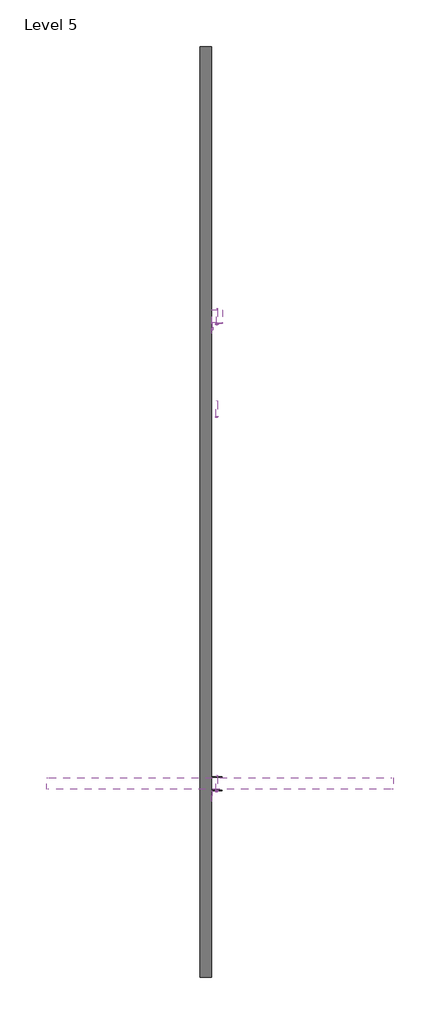
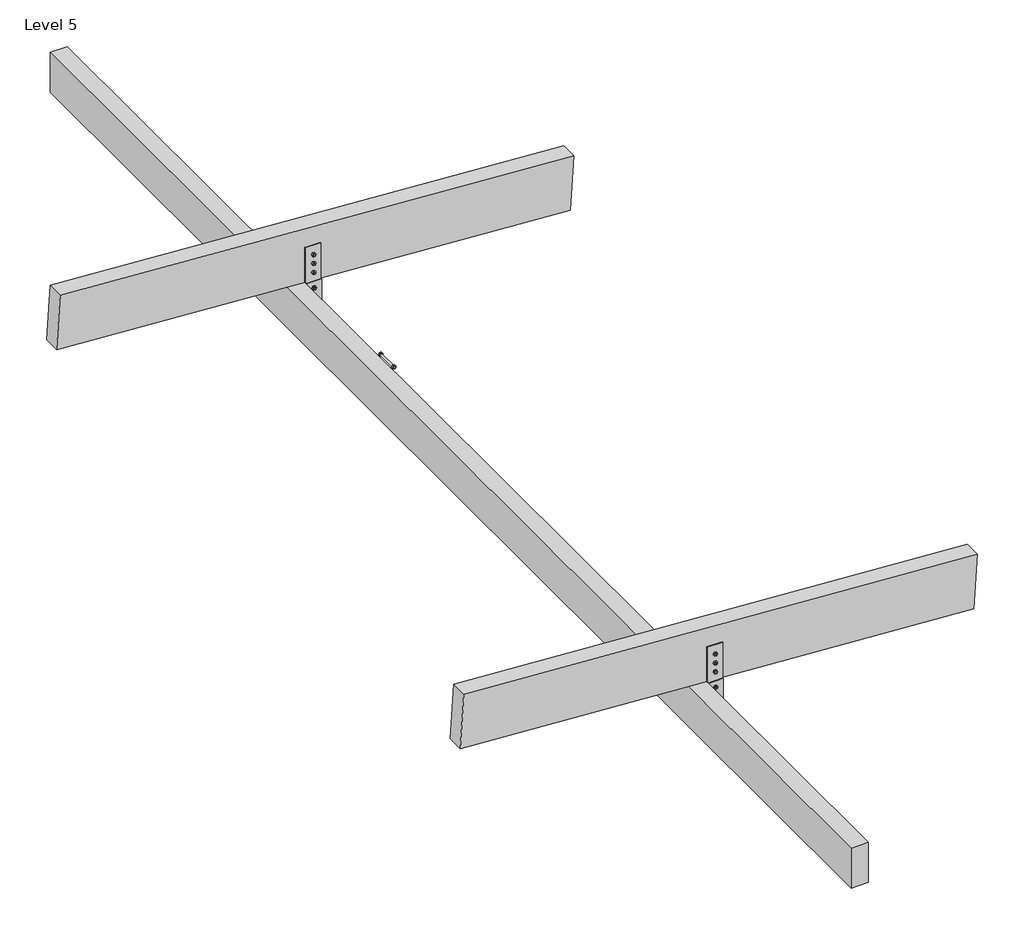
# One storey: 43 proxies.
"""IFC4 building model written with IfcOpenShell, lengths in millimetres."""

import ifcopenshell
import ifcopenshell.guid

model = None  # the IFC model being written
_history = None  # IfcOwnerHistory: only IFC2X3 demands one
_inside = {}  # id of a spatial element -> (the spatial element, [elements in it])
_under = {}  # id of a project, library or spatial element -> (it, [spatial elements below it])
_declared = {}  # id of a project -> (the project, [libraries it declares])
_typed = {}  # id of a type object -> (the type object, [elements of that type])
_made_of = {}  # id of a material, layer set ... -> (it, [elements and type objects made of it])


def new_model(schema):
    """Start an empty IFC model of exactly this schema.

    Asked for "IFC4X3", IfcOpenShell would pick the latest addendum, in which some entities
    have other attributes; the version numbers below select the first issue.
    IFC2X3 requires an IfcOwnerHistory on every rooted entity: one is made here for all.
    """
    global model, _history
    if schema == "IFC4X3":
        model = ifcopenshell.file(schema_version=(4, 3, 0, 0))
    else:
        model = ifcopenshell.file(schema=schema)
    _inside.clear()
    _under.clear()
    _declared.clear()
    _typed.clear()
    _made_of.clear()
    _history = None
    if model.schema == "IFC2X3":
        org = make("IfcOrganization", Name="unknown")
        user = make(
            "IfcPersonAndOrganization",
            ThePerson=make("IfcPerson", FamilyName="unknown"),
            TheOrganization=org,
        )
        app = make(
            "IfcApplication",
            ApplicationDeveloper=org,
            Version="unknown",
            ApplicationFullName="unknown",
            ApplicationIdentifier="unknown",
        )
        _history = make(
            "IfcOwnerHistory",
            OwningUser=user,
            OwningApplication=app,
            ChangeAction="ADDED",
            CreationDate=0,
        )
    return model


def make(cls, **values):
    """One entity of the class cls with the attributes given. An attribute that is None is left unset."""
    return model.create_entity(
        cls, **{name: value for name, value in values.items() if value is not None}
    )


def rooted(cls, **values):
    """An entity with a GlobalId (a new one), such as an element, a storey or a relation."""
    return make(cls, GlobalId=ifcopenshell.guid.new(), OwnerHistory=_history, **values)


def si_unit(unit_type, name, prefix=None):
    """IfcSIUnit, for example si_unit("LENGTHUNIT", "METRE", prefix="MILLI")."""
    return make("IfcSIUnit", UnitType=unit_type, Prefix=prefix, Name=name)


def assignment(units):
    """IfcUnitAssignment: the units of a project."""
    return None if units is None else make("IfcUnitAssignment", Units=units)


def point(xyz):
    """IfcCartesianPoint."""
    return None if xyz is None else make("IfcCartesianPoint", Coordinates=xyz)


def direction(xyz):
    """IfcDirection."""
    return None if xyz is None else make("IfcDirection", DirectionRatios=xyz)


def frame(location, z_axis=None, x_axis=None):
    """IfcAxis2Placement3D, a coordinate frame: its origin and axes. An axis left out is left unset."""
    return make(
        "IfcAxis2Placement3D",
        Location=point(location),
        Axis=direction(z_axis),
        RefDirection=direction(x_axis),
    )


def frame_2d(location, x_axis=None):
    """IfcAxis2Placement2D, a coordinate frame in the plane: its origin and x axis."""
    return make(
        "IfcAxis2Placement2D", Location=point(location), RefDirection=direction(x_axis)
    )


def origin():
    """The frame at (0, 0, 0) with its axes left unset."""
    return frame((0.0, 0.0, 0.0))


def origin_2d():
    """The frame at (0, 0) in the plane with its x axis left unset."""
    return frame_2d((0.0, 0.0))


def place(relative_to, where):
    """IfcLocalPlacement: puts the frame where relative to a parent placement (None: the world)."""
    return make(
        "IfcLocalPlacement", PlacementRelTo=relative_to, RelativePlacement=where
    )


def context(
    kind, dimensions, precision=None, world=None, true_north=None, identifier=None
):
    """IfcGeometricRepresentationContext, for example the 3D "Model" context."""
    return make(
        "IfcGeometricRepresentationContext",
        ContextIdentifier=identifier,
        ContextType=kind,
        CoordinateSpaceDimension=dimensions,
        Precision=precision,
        WorldCoordinateSystem=world,
        TrueNorth=true_north,
    )


def project(units=None, contexts=None):
    """IfcProject with its units and contexts."""
    return rooted(
        "IfcProject",
        Name="project",
        RepresentationContexts=contexts,
        UnitsInContext=assignment(units),
    )


def spatial(cls, under=None, at=None, **own):
    """A site, building, storey or space (cls), placed at a placement, below another one or the project."""
    s = rooted(cls, ObjectPlacement=at, **own)
    if under is not None:
        _under.setdefault(under.id(), (under, []))[1].append(s)
    return s


def polyline(points):
    """IfcPolyline through the points."""
    return make("IfcPolyline", Points=[point(p) for p in points])


def circle_curve(where, radius):
    """IfcCircle in the frame where."""
    return make("IfcCircle", Position=where, Radius=radius)


def trimmed(basis, trim1, trim2, sense, master):
    """IfcTrimmedCurve: the piece of a basis curve between two trims."""
    return make(
        "IfcTrimmedCurve",
        BasisCurve=basis,
        Trim1=trim1,
        Trim2=trim2,
        SenseAgreement=sense,
        MasterRepresentation=master,
    )


def segment(curve, same_sense, transition):
    """IfcCompositeCurveSegment."""
    return make(
        "IfcCompositeCurveSegment",
        Transition=transition,
        SameSense=same_sense,
        ParentCurve=curve,
    )


def composite_curve(segments, self_intersect=None):
    """IfcCompositeCurve: segments joined end to end."""
    return make("IfcCompositeCurve", Segments=segments, SelfIntersect=self_intersect)


def outline(outer, holes=None, kind="AREA"):
    """IfcArbitraryClosedProfileDef: a profile drawn as a closed curve; with holes, ...WithVoids."""
    if holes is None:
        return make("IfcArbitraryClosedProfileDef", ProfileType=kind, OuterCurve=outer)
    return make(
        "IfcArbitraryProfileDefWithVoids",
        ProfileType=kind,
        OuterCurve=outer,
        InnerCurves=holes,
    )


def extrude(swept, where, along, depth):
    """IfcExtrudedAreaSolid: the profile swept, set in the frame where, extruded along a direction by depth."""
    return make(
        "IfcExtrudedAreaSolid",
        SweptArea=swept,
        Position=where,
        ExtrudedDirection=direction(along),
        Depth=depth,
    )


def shape(context_of_items, identifier, shape_type, items):
    """IfcShapeRepresentation: the items that make up one representation, for example the "Body"."""
    return make(
        "IfcShapeRepresentation",
        ContextOfItems=context_of_items,
        RepresentationIdentifier=identifier,
        RepresentationType=shape_type,
        Items=items,
    )


def source(mapping_origin, context_of_items, identifier, shape_type, items):
    """IfcRepresentationMap: a shape defined once, which mapped items show again and again."""
    return make(
        "IfcRepresentationMap",
        MappingOrigin=mapping_origin,
        MappedRepresentation=shape(context_of_items, identifier, shape_type, items),
    )


def transform(
    local_origin,
    x_axis=None,
    y_axis=None,
    z_axis=None,
    scale=None,
    scale2=None,
    scale3=None,
    uniform=True,
):
    """IfcCartesianTransformationOperator3D, or its non-uniform kind. x_axis, y_axis, z_axis: its Axis1, 2, 3."""
    if uniform:
        return make(
            "IfcCartesianTransformationOperator3D",
            Axis1=direction(x_axis),
            Axis2=direction(y_axis),
            LocalOrigin=point(local_origin),
            Scale=scale,
            Axis3=direction(z_axis),
        )
    return make(
        "IfcCartesianTransformationOperator3DnonUniform",
        Axis1=direction(x_axis),
        Axis2=direction(y_axis),
        LocalOrigin=point(local_origin),
        Scale=scale,
        Axis3=direction(z_axis),
        Scale2=scale2,
        Scale3=scale3,
    )


def mapped(mapping_source, mapping_target):
    """IfcMappedItem: shows the shape of a source again, moved by a transform."""
    return make(
        "IfcMappedItem", MappingSource=mapping_source, MappingTarget=mapping_target
    )


def made_of(thing, what):
    """Note that an element or type object is made of a material, layer set ...; save() writes the relation."""
    if what is not None:
        _made_of.setdefault(what.id(), (what, []))[1].append(thing)
    return thing


def element(
    cls,
    number,
    at=None,
    inside=None,
    cuts=None,
    type_object=None,
    material=None,
    context=None,
    identifier="Body",
    shape_type=None,
    held_by="IfcProductDefinitionShape",
    body=None,
    shapes=None,
    **own,
):
    """One element of the class cls, such as IfcWall. Its Tag is "e" and its number.

    at: its placement. inside: the storey or other place that contains it. cuts: it is an
    opening in that element (IfcRelVoidsElement). A single representation is given by context,
    identifier, shape_type and body (its items); several are given by shapes. held_by: the class
    of the entity that holds the representations. save() writes the other relations.
    """
    e = rooted(cls, Tag="e%d" % number, ObjectPlacement=at, **own)
    if body is not None:
        shapes = [shape(context, identifier, shape_type, body)]
    if shapes is not None:
        e.Representation = make(held_by, Representations=shapes)
    if inside is not None:
        _inside.setdefault(inside.id(), (inside, []))[1].append(e)
    if cuts is not None:
        rooted(
            "IfcRelVoidsElement", RelatingBuildingElement=cuts, RelatedOpeningElement=e
        )
    if type_object is not None:
        _typed.setdefault(type_object.id(), (type_object, []))[1].append(e)
    return made_of(e, material)


def aggregate(whole, parts):
    """IfcRelAggregates: a whole, such as a stair, and the parts it consists of."""
    return rooted("IfcRelAggregates", RelatingObject=whole, RelatedObjects=parts)


def save(model, path):
    """Write the relations noted so far, then the file.

    IfcRelAggregates (storeys below a building ...), IfcRelContainedInSpatialStructure (elements
    in a storey), IfcRelDefinesByType, IfcRelAssociatesMaterial and IfcRelDeclares: one each for
    every whole, place, type object, material and project.
    """
    for whole, parts in _under.values():
        aggregate(whole, parts)
    for where, things in _inside.values():
        rooted(
            "IfcRelContainedInSpatialStructure",
            RelatedElements=things,
            RelatingStructure=where,
        )
    for kind, things in _typed.values():
        rooted("IfcRelDefinesByType", RelatedObjects=things, RelatingType=kind)
    for what, things in _made_of.values():
        rooted("IfcRelAssociatesMaterial", RelatedObjects=things, RelatingMaterial=what)
    for by, libraries in _declared.values():
        rooted("IfcRelDeclares", RelatingContext=by, RelatedDefinitions=libraries)
    model.write(path)


def generic_models_108_generic_models_73_f9342414(model_context):
    return source(origin(), model_context, "Body", "SweptSolid", [
        extrude(outline(polyline([(30850.5406612, 271789.525), (30698.1406612, 271789.525), (30698.1406612, 271383.125), (30690.2031612, 271383.125), (30690.2031612, 271797.4625), (30858.4781612, 271797.4625), (30858.4781612, 271383.125), (30850.5406612, 271383.125), (30850.5406612, 271789.525)])), frame((31923.0340778, 0.0, 0.0), z_axis=(1.0, 0.0, 0.0), x_axis=(0.0, 1.0, 0.0)), (0.0, 0.0, 1.0), 127.0),
    ])


def generic_models_142_generic_models_75_680a847f(model_context):
    return source(origin(), model_context, "Body", "SweptSolid", [
        extrude(outline(polyline([(271581.5625, 31979.8726858), (271581.5625, 31996.3704698), (271595.85, 32004.6193618), (271610.1375, 31996.3704698), (271610.1375, 31979.8726858), (271595.85, 31971.6237939), (271581.5625, 31979.8726858)])), frame((0.0, 36311.3770442, 0.0), z_axis=(0.0, 1.0, 0.0), x_axis=(0.0, 0.0, 1.0)), (0.0, 0.0, 1.0), 11.90625),
        extrude(outline(polyline([(271581.5625, 31979.8726858), (271581.5625, 31996.3704698), (271595.85, 32004.6193618), (271610.1375, 31996.3704698), (271610.1375, 31979.8726858), (271595.85, 31971.6237939), (271581.5625, 31979.8726858)])), frame((0.0, 36491.5582942, 0.0), z_axis=(0.0, 1.0, 0.0), x_axis=(0.0, 0.0, 1.0)), (0.0, 0.0, 1.0), 11.90625),
    ])


def generic_models_155_generic_models_75_12a366e2(model_context):
    return source(origin(), model_context, "Body", "SweptSolid", [
        extrude(outline(polyline([(271657.7625, 31979.8726858), (271657.7625, 31996.3704698), (271672.05, 32004.6193618), (271686.3375, 31996.3704698), (271686.3375, 31979.8726858), (271672.05, 31971.6237939), (271657.7625, 31979.8726858)])), frame((0.0, 36311.3770442, 0.0), z_axis=(0.0, 1.0, 0.0), x_axis=(0.0, 0.0, 1.0)), (0.0, 0.0, 1.0), 11.90625),
        extrude(outline(polyline([(271657.7625, 31979.8726858), (271657.7625, 31996.3704698), (271672.05, 32004.6193618), (271686.3375, 31996.3704698), (271686.3375, 31979.8726858), (271672.05, 31971.6237939), (271657.7625, 31979.8726858)])), frame((0.0, 36491.5582942, 0.0), z_axis=(0.0, 1.0, 0.0), x_axis=(0.0, 0.0, 1.0)), (0.0, 0.0, 1.0), 11.90625),
    ])


def generic_models_166_generic_models_73_e2e018fc(model_context):
    return source(origin(), model_context, "Body", "SweptSolid", [
        extrude(outline(polyline([(31923.0340778, 30690.2031612), (31930.9715778, 30690.2031612), (31930.9715778, 30563.2031612), (31923.0340778, 30563.2031612), (31923.0340778, 30690.2031612)])), frame((0.0, 0.0, 271490.7765953), z_axis=(0.0, 0.0, 1.0), x_axis=(1.0, 0.0, 0.0)), (0.0, 0.0, 1.0), 295.5734047),
        extrude(outline(polyline([(31923.0340778, 30985.4781612), (31930.9715778, 30985.4781612), (31930.9715778, 30858.4781612), (31923.0340778, 30858.4781612), (31923.0340778, 30985.4781612)])), frame((0.0, 0.0, 271490.7765953), z_axis=(0.0, 0.0, 1.0), x_axis=(1.0, 0.0, 0.0)), (0.0, 0.0, 1.0), 295.5734047),
        extrude(outline(polyline([(32050.0340778, 30852.1281612), (32050.0340778, 30844.1906612), (31923.0340778, 30844.1906612), (31923.0340778, 30852.1281612), (32050.0340778, 30852.1281612)])), frame((0.0, 0.0, 271797.4625), z_axis=(0.0, 0.0, 1.0), x_axis=(1.0, 0.0, 0.0)), (0.0, 0.0, 1.0), 306.5595065),
        extrude(outline(polyline([(32050.0340778, 30704.4906612), (32050.0340778, 30696.5531612), (31923.0340778, 30696.5531612), (31923.0340778, 30704.4906612), (32050.0340778, 30704.4906612)])), frame((0.0, 0.0, 271797.4625), z_axis=(0.0, 0.0, 1.0), x_axis=(1.0, 0.0, 0.0)), (0.0, 0.0, 1.0), 306.5595065),
    ])


def generic_models_168_generic_models_75_28256fc9(model_context):
    return source(origin(), model_context, "Body", "SweptSolid", [
        extrude(outline(polyline([(271505.3625, 31978.2851858), (271505.3625, 31994.7829698), (271519.65, 32003.0318618), (271533.9375, 31994.7829698), (271533.9375, 31978.2851858), (271519.65, 31970.0362939), (271505.3625, 31978.2851858)])), frame((0.0, 35193.7770442, 0.0), z_axis=(0.0, 1.0, 0.0), x_axis=(0.0, 0.0, 1.0)), (0.0, 0.0, 1.0), 11.90625),
        extrude(outline(polyline([(271505.3625, 31978.2851858), (271505.3625, 31994.7829698), (271519.65, 32003.0318618), (271533.9375, 31994.7829698), (271533.9375, 31978.2851858), (271519.65, 31970.0362939), (271505.3625, 31978.2851858)])), frame((0.0, 35373.9582942, 0.0), z_axis=(0.0, 1.0, 0.0), x_axis=(0.0, 0.0, 1.0)), (0.0, 0.0, 1.0), 11.90625),
    ])


def generic_models_172_generic_models_70_ead40be0(model_context):
    return source(origin(), model_context, "Body", "SweptSolid", [
        extrude(outline(polyline([(0.0, -4165.0140379), (0.0, 0.0), (139.7, 0.0), (139.7, -4165.0140379), (0.0, -4165.0140379)])), frame((29915.3947278, 36337.5707942, 271930.8774594), z_axis=(0.062378286155191545, 0.0, 0.9980525784828879), x_axis=(0.0, 1.0, 0.0)), (0.0, 0.0, 1.0), 457.2),
        extrude(outline(polyline([(0.0, -4165.0140379), (0.0, 0.0), (139.7, 0.0), (139.7, -4165.0140379), (0.0, -4165.0140379)])), frame((29929.8137808, 30704.4906612, 271929.9762686), z_axis=(0.06237828615519167, 0.0, 0.9980525784828879), x_axis=(0.0, 1.0, 0.0)), (0.0, 0.0, 1.0), 457.2),
    ])


def generic_models_173_generic_models_75_790f61a9(model_context):
    return source(origin(), model_context, "Body", "SweptSolid", [
        extrude(outline(polyline([(271581.5625, 31978.2851858), (271581.5625, 31994.7829698), (271595.85, 32003.0318618), (271610.1375, 31994.7829698), (271610.1375, 31978.2851858), (271595.85, 31970.0362939), (271581.5625, 31978.2851858)])), frame((0.0, 35193.7770442, 0.0), z_axis=(0.0, 1.0, 0.0), x_axis=(0.0, 0.0, 1.0)), (0.0, 0.0, 1.0), 11.90625),
        extrude(outline(polyline([(271581.5625, 31978.2851858), (271581.5625, 31994.7829698), (271595.85, 32003.0318618), (271610.1375, 31994.7829698), (271610.1375, 31978.2851858), (271595.85, 31970.0362939), (271581.5625, 31978.2851858)])), frame((0.0, 35373.9582942, 0.0), z_axis=(0.0, 1.0, 0.0), x_axis=(0.0, 0.0, 1.0)), (0.0, 0.0, 1.0), 11.90625),
    ])


def generic_models_174_generic_models_75_63e9463d(model_context):
    return source(origin(), model_context, "Body", "SweptSolid", [
        extrude(outline(polyline([(272027.8220065, 31970.0362939), (272013.5345065, 31978.2851858), (272013.5345065, 31994.7829698), (272027.8220065, 32003.0318618), (272042.1095065, 31994.7829698), (272042.1095065, 31978.2851858), (272027.8220065, 31970.0362939)])), frame((0.0, 30684.6469112, 0.0), z_axis=(0.0, 1.0, 0.0), x_axis=(0.0, 0.0, 1.0)), (0.0, 0.0, 1.0), 11.90625),
        extrude(outline(polyline([(272027.8220065, 31970.0362939), (272013.5345065, 31978.2851858), (272013.5345065, 31994.7829698), (272027.8220065, 32003.0318618), (272042.1095065, 31994.7829698), (272042.1095065, 31978.2851858), (272027.8220065, 31970.0362939)])), frame((0.0, 30852.1281612, 0.0), z_axis=(0.0, 1.0, 0.0), x_axis=(0.0, 0.0, 1.0)), (0.0, 0.0, 1.0), 11.90625),
        extrude(outline(polyline([(271951.6220065, 31970.0362939), (271937.3345065, 31978.2851858), (271937.3345065, 31994.7829698), (271951.6220065, 32003.0318618), (271965.9095065, 31994.7829698), (271965.9095065, 31978.2851858), (271951.6220065, 31970.0362939)])), frame((0.0, 30684.6469112, 0.0), z_axis=(0.0, 1.0, 0.0), x_axis=(0.0, 0.0, 1.0)), (0.0, 0.0, 1.0), 11.90625),
        extrude(outline(polyline([(271951.6220065, 31970.0362939), (271937.3345065, 31978.2851858), (271937.3345065, 31994.7829698), (271951.6220065, 32003.0318618), (271965.9095065, 31994.7829698), (271965.9095065, 31978.2851858), (271951.6220065, 31970.0362939)])), frame((0.0, 30852.1281612, 0.0), z_axis=(0.0, 1.0, 0.0), x_axis=(0.0, 0.0, 1.0)), (0.0, 0.0, 1.0), 11.90625),
        extrude(outline(polyline([(271875.4220065, 31970.0362939), (271861.1345065, 31978.2851858), (271861.1345065, 31994.7829698), (271875.4220065, 32003.0318618), (271889.7095065, 31994.7829698), (271889.7095065, 31978.2851858), (271875.4220065, 31970.0362939)])), frame((0.0, 30684.6469112, 0.0), z_axis=(0.0, 1.0, 0.0), x_axis=(0.0, 0.0, 1.0)), (0.0, 0.0, 1.0), 11.90625),
        extrude(outline(polyline([(271875.4220065, 31970.0362939), (271861.1345065, 31978.2851858), (271861.1345065, 31994.7829698), (271875.4220065, 32003.0318618), (271889.7095065, 31994.7829698), (271889.7095065, 31978.2851858), (271875.4220065, 31970.0362939)])), frame((0.0, 30852.1281612, 0.0), z_axis=(0.0, 1.0, 0.0), x_axis=(0.0, 0.0, 1.0)), (0.0, 0.0, 1.0), 11.90625),
    ])


def generic_models_175_generic_models_75_4c8c2855(model_context):
    return source(origin(), model_context, "Body", "SweptSolid", [
        extrude(outline(polyline([(271657.7625, 31978.2851858), (271657.7625, 31994.7829698), (271672.05, 32003.0318618), (271686.3375, 31994.7829698), (271686.3375, 31978.2851858), (271672.05, 31970.0362939), (271657.7625, 31978.2851858)])), frame((0.0, 35193.7770442, 0.0), z_axis=(0.0, 1.0, 0.0), x_axis=(0.0, 0.0, 1.0)), (0.0, 0.0, 1.0), 11.90625),
        extrude(outline(polyline([(271657.7625, 31978.2851858), (271657.7625, 31994.7829698), (271672.05, 32003.0318618), (271686.3375, 31994.7829698), (271686.3375, 31978.2851858), (271672.05, 31970.0362939), (271657.7625, 31978.2851858)])), frame((0.0, 35373.9582942, 0.0), z_axis=(0.0, 1.0, 0.0), x_axis=(0.0, 0.0, 1.0)), (0.0, 0.0, 1.0), 11.90625),
    ])


def generic_models_176_generic_models_75_eb76e51d(model_context):
    return source(origin(), model_context, "Body", "SweptSolid", [
        extrude(outline(polyline([(271733.9625, 31978.2851858), (271733.9625, 31994.7829698), (271748.25, 32003.0318618), (271762.5375, 31994.7829698), (271762.5375, 31978.2851858), (271748.25, 31970.0362939), (271733.9625, 31978.2851858)])), frame((0.0, 35193.7770442, 0.0), z_axis=(0.0, 1.0, 0.0), x_axis=(0.0, 0.0, 1.0)), (0.0, 0.0, 1.0), 11.90625),
        extrude(outline(polyline([(271733.9625, 31978.2851858), (271733.9625, 31994.7829698), (271748.25, 32003.0318618), (271762.5375, 31994.7829698), (271762.5375, 31978.2851858), (271748.25, 31970.0362939), (271733.9625, 31978.2851858)])), frame((0.0, 35373.9582942, 0.0), z_axis=(0.0, 1.0, 0.0), x_axis=(0.0, 0.0, 1.0)), (0.0, 0.0, 1.0), 11.90625),
    ])


def generic_models_179_generic_models_75_1166544c(model_context):
    return source(origin(), model_context, "Body", "SweptSolid", [
        extrude(outline(polyline([(271733.9625, 31979.8726858), (271733.9625, 31996.3704698), (271748.25, 32004.6193618), (271762.5375, 31996.3704698), (271762.5375, 31979.8726858), (271748.25, 31971.6237939), (271733.9625, 31979.8726858)])), frame((0.0, 36311.3770442, 0.0), z_axis=(0.0, 1.0, 0.0), x_axis=(0.0, 0.0, 1.0)), (0.0, 0.0, 1.0), 11.90625),
        extrude(outline(polyline([(271733.9625, 31979.8726858), (271733.9625, 31996.3704698), (271748.25, 32004.6193618), (271762.5375, 31996.3704698), (271762.5375, 31979.8726858), (271748.25, 31971.6237939), (271733.9625, 31979.8726858)])), frame((0.0, 36491.5582942, 0.0), z_axis=(0.0, 1.0, 0.0), x_axis=(0.0, 0.0, 1.0)), (0.0, 0.0, 1.0), 11.90625),
    ])


def generic_models_197_generic_models_75_ac2514aa(model_context):
    return source(origin(), model_context, "Body", "SweptSolid", [
        extrude(outline(polyline([(271505.3625, 31978.2851858), (271505.3625, 31994.7829698), (271519.65, 32003.0318618), (271533.9375, 31994.7829698), (271533.9375, 31978.2851858), (271519.65, 31970.0362939), (271505.3625, 31978.2851858)])), frame((0.0, 30678.2969112, 0.0), z_axis=(0.0, 1.0, 0.0), x_axis=(0.0, 0.0, 1.0)), (0.0, 0.0, 1.0), 11.90625),
        extrude(outline(polyline([(271505.3625, 31978.2851858), (271505.3625, 31994.7829698), (271519.65, 32003.0318618), (271533.9375, 31994.7829698), (271533.9375, 31978.2851858), (271519.65, 31970.0362939), (271505.3625, 31978.2851858)])), frame((0.0, 30858.4781612, 0.0), z_axis=(0.0, 1.0, 0.0), x_axis=(0.0, 0.0, 1.0)), (0.0, 0.0, 1.0), 11.90625),
    ])


def generic_models_199_generic_models_75_efedec74(model_context):
    return source(origin(), model_context, "Body", "SweptSolid", [
        extrude(outline(polyline([(271581.5625, 31978.2851858), (271581.5625, 31994.7829698), (271595.85, 32003.0318618), (271610.1375, 31994.7829698), (271610.1375, 31978.2851858), (271595.85, 31970.0362939), (271581.5625, 31978.2851858)])), frame((0.0, 30678.2969112, 0.0), z_axis=(0.0, 1.0, 0.0), x_axis=(0.0, 0.0, 1.0)), (0.0, 0.0, 1.0), 11.90625),
        extrude(outline(polyline([(271581.5625, 31978.2851858), (271581.5625, 31994.7829698), (271595.85, 32003.0318618), (271610.1375, 31994.7829698), (271610.1375, 31978.2851858), (271595.85, 31970.0362939), (271581.5625, 31978.2851858)])), frame((0.0, 30858.4781612, 0.0), z_axis=(0.0, 1.0, 0.0), x_axis=(0.0, 0.0, 1.0)), (0.0, 0.0, 1.0), 11.90625),
    ])


def generic_models_203_generic_models_75_2103832a(model_context):
    return source(origin(), model_context, "Body", "SweptSolid", [
        extrude(outline(polyline([(30612.3964892, 271527.9099609), (30626.7031612, 271536.1699219), (30641.0098332, 271527.9099609), (30641.0098332, 271511.3900391), (30626.7031612, 271503.1300781), (30612.3964892, 271511.3900391), (30612.3964892, 271527.9099609)])), frame((31930.9715778, 0.0, 0.0), z_axis=(1.0, 0.0, 0.0), x_axis=(0.0, 1.0, 0.0)), (0.0, 0.0, 1.0), 11.90625),
        extrude(outline(polyline([(30612.3964892, 271604.1099609), (30626.7031612, 271612.3699219), (30641.0098332, 271604.1099609), (30641.0098332, 271587.5900391), (30626.7031612, 271579.3300781), (30612.3964892, 271587.5900391), (30612.3964892, 271604.1099609)])), frame((31930.9715778, 0.0, 0.0), z_axis=(1.0, 0.0, 0.0), x_axis=(0.0, 1.0, 0.0)), (0.0, 0.0, 1.0), 11.90625),
        extrude(outline(polyline([(30612.3964892, 271680.3099609), (30626.7031612, 271688.5699219), (30641.0098332, 271680.3099609), (30641.0098332, 271663.7900391), (30626.7031612, 271655.5300781), (30612.3964892, 271663.7900391), (30612.3964892, 271680.3099609)])), frame((31930.9715778, 0.0, 0.0), z_axis=(1.0, 0.0, 0.0), x_axis=(0.0, 1.0, 0.0)), (0.0, 0.0, 1.0), 11.90625),
        extrude(outline(polyline([(30612.3964892, 271756.5099609), (30626.7031612, 271764.7699219), (30641.0098332, 271756.5099609), (30641.0098332, 271739.9900391), (30626.7031612, 271731.7300781), (30612.3964892, 271739.9900391), (30612.3964892, 271756.5099609)])), frame((31930.9715778, 0.0, 0.0), z_axis=(1.0, 0.0, 0.0), x_axis=(0.0, 1.0, 0.0)), (0.0, 0.0, 1.0), 11.90625),
        extrude(outline(polyline([(30907.6714892, 271527.9099609), (30921.9781612, 271536.1699219), (30936.2848332, 271527.9099609), (30936.2848332, 271511.3900391), (30921.9781612, 271503.1300781), (30907.6714892, 271511.3900391), (30907.6714892, 271527.9099609)])), frame((31930.9715778, 0.0, 0.0), z_axis=(1.0, 0.0, 0.0), x_axis=(0.0, 1.0, 0.0)), (0.0, 0.0, 1.0), 11.90625),
        extrude(outline(polyline([(30907.6714892, 271604.1099609), (30921.9781612, 271612.3699219), (30936.2848332, 271604.1099609), (30936.2848332, 271587.5900391), (30921.9781612, 271579.3300781), (30907.6714892, 271587.5900391), (30907.6714892, 271604.1099609)])), frame((31930.9715778, 0.0, 0.0), z_axis=(1.0, 0.0, 0.0), x_axis=(0.0, 1.0, 0.0)), (0.0, 0.0, 1.0), 11.90625),
        extrude(outline(polyline([(30907.6714892, 271680.3099609), (30921.9781612, 271688.5699219), (30936.2848332, 271680.3099609), (30936.2848332, 271663.7900391), (30921.9781612, 271655.5300781), (30907.6714892, 271663.7900391), (30907.6714892, 271680.3099609)])), frame((31930.9715778, 0.0, 0.0), z_axis=(1.0, 0.0, 0.0), x_axis=(0.0, 1.0, 0.0)), (0.0, 0.0, 1.0), 11.90625),
        extrude(outline(polyline([(35158.6810781, 271681.575), (35158.6810781, 271662.525), (35142.1832942, 271653.0), (35125.6855103, 271662.525), (35125.6855103, 271681.575), (35142.1832942, 271691.1), (35158.6810781, 271681.575)])), frame((31930.9715778, 0.0, 0.0), z_axis=(1.0, 0.0, 0.0), x_axis=(0.0, 1.0, 0.0)), (0.0, 0.0, 1.0), 11.90625),
        extrude(outline(polyline([(35158.6810781, 271605.375), (35158.6810781, 271586.325), (35142.1832942, 271576.8), (35125.6855103, 271586.325), (35125.6855103, 271605.375), (35142.1832942, 271614.9), (35158.6810781, 271605.375)])), frame((31930.9715778, 0.0, 0.0), z_axis=(1.0, 0.0, 0.0), x_axis=(0.0, 1.0, 0.0)), (0.0, 0.0, 1.0), 11.90625),
        extrude(outline(polyline([(36571.5560781, 271529.175), (36571.5560781, 271510.125), (36555.0582942, 271500.6), (36538.5605103, 271510.125), (36538.5605103, 271529.175), (36555.0582942, 271538.7), (36571.5560781, 271529.175)])), frame((31930.9715778, 0.0, 0.0), z_axis=(1.0, 0.0, 0.0), x_axis=(0.0, 1.0, 0.0)), (0.0, 0.0, 1.0), 11.90625),
        extrude(outline(polyline([(36571.5560781, 271605.375), (36571.5560781, 271586.325), (36555.0582942, 271576.8), (36538.5605103, 271586.325), (36538.5605103, 271605.375), (36555.0582942, 271614.9), (36571.5560781, 271605.375)])), frame((31930.9715778, 0.0, 0.0), z_axis=(1.0, 0.0, 0.0), x_axis=(0.0, 1.0, 0.0)), (0.0, 0.0, 1.0), 11.90625),
        extrude(outline(polyline([(36571.5560781, 271681.575), (36571.5560781, 271662.525), (36555.0582942, 271653.0), (36538.5605103, 271662.525), (36538.5605103, 271681.575), (36555.0582942, 271691.1), (36571.5560781, 271681.575)])), frame((31930.9715778, 0.0, 0.0), z_axis=(1.0, 0.0, 0.0), x_axis=(0.0, 1.0, 0.0)), (0.0, 0.0, 1.0), 11.90625),
        extrude(outline(polyline([(36571.5560781, 271757.775), (36571.5560781, 271738.725), (36555.0582942, 271729.2), (36538.5605103, 271738.725), (36538.5605103, 271757.775), (36555.0582942, 271767.3), (36571.5560781, 271757.775)])), frame((31930.9715778, 0.0, 0.0), z_axis=(1.0, 0.0, 0.0), x_axis=(0.0, 1.0, 0.0)), (0.0, 0.0, 1.0), 11.90625),
        extrude(outline(polyline([(36276.2810781, 271529.175), (36276.2810781, 271510.125), (36259.7832942, 271500.6), (36243.2855103, 271510.125), (36243.2855103, 271529.175), (36259.7832942, 271538.7), (36276.2810781, 271529.175)])), frame((31930.9715778, 0.0, 0.0), z_axis=(1.0, 0.0, 0.0), x_axis=(0.0, 1.0, 0.0)), (0.0, 0.0, 1.0), 11.90625),
        extrude(outline(polyline([(36276.2810781, 271605.375), (36276.2810781, 271586.325), (36259.7832942, 271576.8), (36243.2855103, 271586.325), (36243.2855103, 271605.375), (36259.7832942, 271614.9), (36276.2810781, 271605.375)])), frame((31930.9715778, 0.0, 0.0), z_axis=(1.0, 0.0, 0.0), x_axis=(0.0, 1.0, 0.0)), (0.0, 0.0, 1.0), 11.90625),
        extrude(outline(polyline([(36276.2810781, 271681.575), (36276.2810781, 271662.525), (36259.7832942, 271653.0), (36243.2855103, 271662.525), (36243.2855103, 271681.575), (36259.7832942, 271691.1), (36276.2810781, 271681.575)])), frame((31930.9715778, 0.0, 0.0), z_axis=(1.0, 0.0, 0.0), x_axis=(0.0, 1.0, 0.0)), (0.0, 0.0, 1.0), 11.90625),
        extrude(outline(polyline([(36276.2810781, 271757.775), (36276.2810781, 271738.725), (36259.7832942, 271729.2), (36243.2855103, 271738.725), (36243.2855103, 271757.775), (36259.7832942, 271767.3), (36276.2810781, 271757.775)])), frame((31930.9715778, 0.0, 0.0), z_axis=(1.0, 0.0, 0.0), x_axis=(0.0, 1.0, 0.0)), (0.0, 0.0, 1.0), 11.90625),
        extrude(outline(polyline([(35453.9560781, 271529.175), (35453.9560781, 271510.125), (35437.4582942, 271500.6), (35420.9605103, 271510.125), (35420.9605103, 271529.175), (35437.4582942, 271538.7), (35453.9560781, 271529.175)])), frame((31930.9715778, 0.0, 0.0), z_axis=(1.0, 0.0, 0.0), x_axis=(0.0, 1.0, 0.0)), (0.0, 0.0, 1.0), 11.90625),
        extrude(outline(polyline([(35453.9560781, 271605.375), (35453.9560781, 271586.325), (35437.4582942, 271576.8), (35420.9605103, 271586.325), (35420.9605103, 271605.375), (35437.4582942, 271614.9), (35453.9560781, 271605.375)])), frame((31930.9715778, 0.0, 0.0), z_axis=(1.0, 0.0, 0.0), x_axis=(0.0, 1.0, 0.0)), (0.0, 0.0, 1.0), 11.90625),
        extrude(outline(polyline([(35453.9560781, 271681.575), (35453.9560781, 271662.525), (35437.4582942, 271653.0), (35420.9605103, 271662.525), (35420.9605103, 271681.575), (35437.4582942, 271691.1), (35453.9560781, 271681.575)])), frame((31930.9715778, 0.0, 0.0), z_axis=(1.0, 0.0, 0.0), x_axis=(0.0, 1.0, 0.0)), (0.0, 0.0, 1.0), 11.90625),
        extrude(outline(polyline([(35453.9560781, 271757.775), (35453.9560781, 271738.725), (35437.4582942, 271729.2), (35420.9605103, 271738.725), (35420.9605103, 271757.775), (35437.4582942, 271767.3), (35453.9560781, 271757.775)])), frame((31930.9715778, 0.0, 0.0), z_axis=(1.0, 0.0, 0.0), x_axis=(0.0, 1.0, 0.0)), (0.0, 0.0, 1.0), 11.90625),
        extrude(outline(polyline([(35158.6810781, 271529.175), (35158.6810781, 271510.125), (35142.1832942, 271500.6), (35125.6855103, 271510.125), (35125.6855103, 271529.175), (35142.1832942, 271538.7), (35158.6810781, 271529.175)])), frame((31930.9715778, 0.0, 0.0), z_axis=(1.0, 0.0, 0.0), x_axis=(0.0, 1.0, 0.0)), (0.0, 0.0, 1.0), 11.90625),
        extrude(outline(polyline([(35158.6810781, 271757.775), (35158.6810781, 271738.725), (35142.1832942, 271729.2), (35125.6855103, 271738.725), (35125.6855103, 271757.775), (35142.1832942, 271767.3), (35158.6810781, 271757.775)])), frame((31930.9715778, 0.0, 0.0), z_axis=(1.0, 0.0, 0.0), x_axis=(0.0, 1.0, 0.0)), (0.0, 0.0, 1.0), 11.90625),
        extrude(outline(polyline([(30907.6714892, 271756.5099609), (30921.9781612, 271764.7699219), (30936.2848332, 271756.5099609), (30936.2848332, 271739.9900391), (30921.9781612, 271731.7300781), (30907.6714892, 271739.9900391), (30907.6714892, 271756.5099609)])), frame((31930.9715778, 0.0, 0.0), z_axis=(1.0, 0.0, 0.0), x_axis=(0.0, 1.0, 0.0)), (0.0, 0.0, 1.0), 11.90625),
    ])


def generic_models_207_generic_models_75_89b729dd(model_context):
    return source(origin(), model_context, "Body", "SweptSolid", [
        extrude(outline(polyline([(271657.7625, 31978.2851858), (271657.7625, 31994.7829698), (271672.05, 32003.0318618), (271686.3375, 31994.7829698), (271686.3375, 31978.2851858), (271672.05, 31970.0362939), (271657.7625, 31978.2851858)])), frame((0.0, 30678.2969112, 0.0), z_axis=(0.0, 1.0, 0.0), x_axis=(0.0, 0.0, 1.0)), (0.0, 0.0, 1.0), 11.90625),
        extrude(outline(polyline([(271657.7625, 31978.2851858), (271657.7625, 31994.7829698), (271672.05, 32003.0318618), (271686.3375, 31994.7829698), (271686.3375, 31978.2851858), (271672.05, 31970.0362939), (271657.7625, 31978.2851858)])), frame((0.0, 30858.4781612, 0.0), z_axis=(0.0, 1.0, 0.0), x_axis=(0.0, 0.0, 1.0)), (0.0, 0.0, 1.0), 11.90625),
    ])


def generic_models_211_generic_models_75_f9ca25a0(model_context):
    return source(origin(), model_context, "Body", "SweptSolid", [
        extrude(outline(polyline([(271733.9625, 31978.2851858), (271733.9625, 31994.7829698), (271748.25, 32003.0318618), (271762.5375, 31994.7829698), (271762.5375, 31978.2851858), (271748.25, 31970.0362939), (271733.9625, 31978.2851858)])), frame((0.0, 30678.2969112, 0.0), z_axis=(0.0, 1.0, 0.0), x_axis=(0.0, 0.0, 1.0)), (0.0, 0.0, 1.0), 11.90625),
        extrude(outline(polyline([(271733.9625, 31978.2851858), (271733.9625, 31994.7829698), (271748.25, 32003.0318618), (271762.5375, 31994.7829698), (271762.5375, 31978.2851858), (271748.25, 31970.0362939), (271733.9625, 31978.2851858)])), frame((0.0, 30858.4781612, 0.0), z_axis=(0.0, 1.0, 0.0), x_axis=(0.0, 0.0, 1.0)), (0.0, 0.0, 1.0), 11.90625),
    ])


def generic_models_239_generic_models_75_548b8a24(model_context):
    return source(origin(), model_context, "Body", "SweptSolid", [
        extrude(outline(polyline([(272027.8220065, 31971.6237939), (272013.5345065, 31979.8726858), (272013.5345065, 31996.3704698), (272027.8220065, 32004.6193618), (272042.1095065, 31996.3704698), (272042.1095065, 31979.8726858), (272027.8220065, 31971.6237939)])), frame((0.0, 36317.7270442, 0.0), z_axis=(0.0, 1.0, 0.0), x_axis=(0.0, 0.0, 1.0)), (0.0, 0.0, 1.0), 11.90625),
        extrude(outline(polyline([(272027.8220065, 31971.6237939), (272013.5345065, 31979.8726858), (272013.5345065, 31996.3704698), (272027.8220065, 32004.6193618), (272042.1095065, 31996.3704698), (272042.1095065, 31979.8726858), (272027.8220065, 31971.6237939)])), frame((0.0, 36485.2082942, 0.0), z_axis=(0.0, 1.0, 0.0), x_axis=(0.0, 0.0, 1.0)), (0.0, 0.0, 1.0), 11.90625),
        extrude(outline(polyline([(271951.6220065, 31971.6237939), (271937.3345065, 31979.8726858), (271937.3345065, 31996.3704698), (271951.6220065, 32004.6193618), (271965.9095065, 31996.3704698), (271965.9095065, 31979.8726858), (271951.6220065, 31971.6237939)])), frame((0.0, 36317.7270442, 0.0), z_axis=(0.0, 1.0, 0.0), x_axis=(0.0, 0.0, 1.0)), (0.0, 0.0, 1.0), 11.90625),
        extrude(outline(polyline([(271951.6220065, 31971.6237939), (271937.3345065, 31979.8726858), (271937.3345065, 31996.3704698), (271951.6220065, 32004.6193618), (271965.9095065, 31996.3704698), (271965.9095065, 31979.8726858), (271951.6220065, 31971.6237939)])), frame((0.0, 36485.2082942, 0.0), z_axis=(0.0, 1.0, 0.0), x_axis=(0.0, 0.0, 1.0)), (0.0, 0.0, 1.0), 11.90625),
        extrude(outline(polyline([(271875.4220065, 31971.6237939), (271861.1345065, 31979.8726858), (271861.1345065, 31996.3704698), (271875.4220065, 32004.6193618), (271889.7095065, 31996.3704698), (271889.7095065, 31979.8726858), (271875.4220065, 31971.6237939)])), frame((0.0, 36317.7270442, 0.0), z_axis=(0.0, 1.0, 0.0), x_axis=(0.0, 0.0, 1.0)), (0.0, 0.0, 1.0), 11.90625),
        extrude(outline(polyline([(271875.4220065, 31971.6237939), (271861.1345065, 31979.8726858), (271861.1345065, 31996.3704698), (271875.4220065, 32004.6193618), (271889.7095065, 31996.3704698), (271889.7095065, 31979.8726858), (271875.4220065, 31971.6237939)])), frame((0.0, 36485.2082942, 0.0), z_axis=(0.0, 1.0, 0.0), x_axis=(0.0, 0.0, 1.0)), (0.0, 0.0, 1.0), 11.90625),
    ])


def generic_models_272_generic_models_73_2b91d6a2(model_context):
    return source(origin(), model_context, "Body", "SweptSolid", [
        extrude(outline(polyline([(36483.6207942, 271789.525), (36331.2207942, 271789.525), (36331.2207942, 271481.55), (36323.2832942, 271481.55), (36323.2832942, 271797.4625), (36491.5582942, 271797.4625), (36491.5582942, 271481.55), (36483.6207942, 271481.55), (36483.6207942, 271789.525)])), frame((31930.9715778, 0.0, 0.0), z_axis=(1.0, 0.0, 0.0), x_axis=(0.0, 1.0, 0.0)), (0.0, 0.0, 1.0), 122.2375),
    ])


def generic_models_70_generic_models_70_98601c22(model_context):
    return source(origin(), model_context, "Body", "SweptSolid", [
        extrude(outline(polyline([(31923.0340778, 39663.9958903), (31923.0340778, 28437.6872112), (31783.3340778, 28437.6872112), (31783.3340778, 39663.9958903), (31923.0340778, 39663.9958903)])), frame((0.0, 0.0, 271462.5), z_axis=(0.0, 0.0, 1.0), x_axis=(1.0, 0.0, 0.0)), (0.0, 0.0, 1.0), 342.9),
    ])


def generic_models_73_generic_models_73_00176bc8(model_context):
    return source(origin(), model_context, "Body", "SweptSolid", [
        extrude(outline(polyline([(31923.0340778, 36329.6332942), (31930.9715778, 36329.6332942), (31930.9715778, 36204.2207942), (31923.0340778, 36204.2207942), (31923.0340778, 36329.6332942)])), frame((0.0, 0.0, 271481.55), z_axis=(0.0, 0.0, 1.0), x_axis=(1.0, 0.0, 0.0)), (0.0, 0.0, 1.0), 304.8),
        extrude(outline(polyline([(31923.0340778, 36610.6207942), (31930.9715778, 36610.6207942), (31930.9715778, 36485.2082942), (31923.0340778, 36485.2082942), (31923.0340778, 36610.6207942)])), frame((0.0, 0.0, 271481.55), z_axis=(0.0, 0.0, 1.0), x_axis=(1.0, 0.0, 0.0)), (0.0, 0.0, 1.0), 304.8),
        extrude(outline(polyline([(32050.0340778, 36485.2082942), (32050.0340778, 36477.2707942), (31923.0340778, 36477.2707942), (31923.0340778, 36485.2082942), (32050.0340778, 36485.2082942)])), frame((0.0, 0.0, 271797.4625), z_axis=(0.0, 0.0, 1.0), x_axis=(1.0, 0.0, 0.0)), (0.0, 0.0, 1.0), 306.5595065),
        extrude(outline(polyline([(32050.0340778, 36337.5707942), (32050.0340778, 36329.6332942), (31923.0340778, 36329.6332942), (31923.0340778, 36337.5707942), (32050.0340778, 36337.5707942)])), frame((0.0, 0.0, 271797.4625), z_axis=(0.0, 0.0, 1.0), x_axis=(1.0, 0.0, 0.0)), (0.0, 0.0, 1.0), 306.5595065),
    ])


def generic_models_79_generic_models_75_cd3e6485(model_context):
    return source(origin(), model_context, "Body", "SweptSolid", [
        extrude(outline(polyline([(271505.3625, 31979.8726858), (271505.3625, 31996.3704698), (271519.65, 32004.6193618), (271533.9375, 31996.3704698), (271533.9375, 31979.8726858), (271519.65, 31971.6237939), (271505.3625, 31979.8726858)])), frame((0.0, 36311.3770442, 0.0), z_axis=(0.0, 1.0, 0.0), x_axis=(0.0, 0.0, 1.0)), (0.0, 0.0, 1.0), 11.90625),
        extrude(outline(polyline([(271505.3625, 31979.8726858), (271505.3625, 31996.3704698), (271519.65, 32004.6193618), (271533.9375, 31996.3704698), (271533.9375, 31979.8726858), (271519.65, 31971.6237939), (271505.3625, 31979.8726858)])), frame((0.0, 36491.5582942, 0.0), z_axis=(0.0, 1.0, 0.0), x_axis=(0.0, 0.0, 1.0)), (0.0, 0.0, 1.0), 11.90625),
    ])


def rod_rod_9b827da6(model_context):
    return source(origin(), model_context, "Body", "SweptSolid", [
        extrude(outline(composite_curve([segment(trimmed(circle_curve(origin_2d(), 8.1359375), [point((0.0, 8.1359375))], [point((0.0, -8.1359375))], False, "CARTESIAN"), True, "CONTINUOUS"), segment(trimmed(circle_curve(origin_2d(), 8.1359375), [point((0.0, -8.1359375))], [point((0.0, 8.1359375))], False, "CARTESIAN"), True, "CONTINUOUS")], self_intersect=False)), frame((0.0, -152.4, 0.0), z_axis=(0.0, 1.0, 0.0), x_axis=(0.0, 0.0, 1.0)), (0.0, 0.0, 1.0), 184.15),
    ])


def rod_rod_8_5da43aea(model_context):
    return source(origin(), model_context, "Body", "SweptSolid", [
        extrude(outline(composite_curve([segment(trimmed(circle_curve(origin_2d(), 8.1359375), [point((0.0, 8.1359375))], [point((0.0, -8.1359375))], False, "CARTESIAN"), True, "CONTINUOUS"), segment(trimmed(circle_curve(origin_2d(), 8.1359375), [point((0.0, -8.1359375))], [point((0.0, 8.1359375))], False, "CARTESIAN"), True, "CONTINUOUS")], self_intersect=False)), frame((0.0, -152.4, 0.0), z_axis=(0.0, 1.0, 0.0), x_axis=(0.0, 0.0, 1.0)), (0.0, 0.0, 1.0), 203.2),
    ])


model = new_model("IFC4")

# Units and contexts
model_context = context("Model", 3, world=origin())
ifc_project = project(units=[si_unit("LENGTHUNIT", "METRE", prefix="MILLI")], contexts=[model_context])

# Site, building, storey
site = spatial("IfcSite", under=ifc_project)
building = spatial("IfcBuilding", under=site)
storey = spatial("IfcBuildingStorey", under=building, Name="Level 5", Elevation=270275.3011428)

# Proxies
placement = place(None, origin())
generic_models_108_generic_models_73_shape = generic_models_108_generic_models_73_f9342414(model_context)
element("IfcBuildingElementProxy", 1, Name="Generic Models 108 : Generic Models 73", ObjectType="Generic Models 108 : Generic Models 73", at=placement, inside=storey, context=model_context, shape_type="MappedRepresentation", body=[
    mapped(generic_models_108_generic_models_73_shape, transform((0.0, 0.0, 0.0), x_axis=(1.0, 0.0, 0.0), y_axis=(0.0, 1.0, 0.0), z_axis=(0.0, 0.0, 1.0))),
])
generic_models_142_generic_models_75_shape = generic_models_142_generic_models_75_680a847f(model_context)
element("IfcBuildingElementProxy", 2, Name="Generic Models 142 : Generic Models 75", ObjectType="Generic Models 142 : Generic Models 75", at=placement, inside=storey, context=model_context, shape_type="MappedRepresentation", body=[
    mapped(generic_models_142_generic_models_75_shape, transform((0.0, 0.0, 0.0), x_axis=(1.0, 0.0, 0.0), y_axis=(0.0, 1.0, 0.0), z_axis=(0.0, 0.0, 1.0))),
])
generic_models_155_generic_models_75_shape = generic_models_155_generic_models_75_12a366e2(model_context)
element("IfcBuildingElementProxy", 3, Name="Generic Models 155 : Generic Models 75", ObjectType="Generic Models 155 : Generic Models 75", at=placement, inside=storey, context=model_context, shape_type="MappedRepresentation", body=[
    mapped(generic_models_155_generic_models_75_shape, transform((0.0, 0.0, 0.0), x_axis=(1.0, 0.0, 0.0), y_axis=(0.0, 1.0, 0.0), z_axis=(0.0, 0.0, 1.0))),
])
generic_models_166_generic_models_73_shape = generic_models_166_generic_models_73_e2e018fc(model_context)
element("IfcBuildingElementProxy", 4, Name="Generic Models 166 : Generic Models 73", ObjectType="Generic Models 166 : Generic Models 73", at=placement, inside=storey, context=model_context, shape_type="MappedRepresentation", body=[
    mapped(generic_models_166_generic_models_73_shape, transform((0.0, 0.0, 0.0), x_axis=(1.0, 0.0, 0.0), y_axis=(0.0, 1.0, 0.0), z_axis=(0.0, 0.0, 1.0))),
])
generic_models_168_generic_models_75_shape = generic_models_168_generic_models_75_28256fc9(model_context)
element("IfcBuildingElementProxy", 5, Name="Generic Models 168 : Generic Models 75", ObjectType="Generic Models 168 : Generic Models 75", at=placement, inside=storey, context=model_context, shape_type="MappedRepresentation", body=[
    mapped(generic_models_168_generic_models_75_shape, transform((0.0, 0.0, 0.0), x_axis=(1.0, 0.0, 0.0), y_axis=(0.0, 1.0, 0.0), z_axis=(0.0, 0.0, 1.0))),
])
generic_models_172_generic_models_70_shape = generic_models_172_generic_models_70_ead40be0(model_context)
element("IfcBuildingElementProxy", 6, Name="Generic Models 172 : Generic Models 70", ObjectType="Generic Models 172 : Generic Models 70", at=placement, inside=storey, context=model_context, shape_type="MappedRepresentation", body=[
    mapped(generic_models_172_generic_models_70_shape, transform((0.0, 0.0, 0.0), x_axis=(1.0, 0.0, 0.0), y_axis=(0.0, 1.0, 0.0), z_axis=(0.0, 0.0, 1.0))),
])
generic_models_173_generic_models_75_shape = generic_models_173_generic_models_75_790f61a9(model_context)
element("IfcBuildingElementProxy", 7, Name="Generic Models 173 : Generic Models 75", ObjectType="Generic Models 173 : Generic Models 75", at=placement, inside=storey, context=model_context, shape_type="MappedRepresentation", body=[
    mapped(generic_models_173_generic_models_75_shape, transform((0.0, 0.0, 0.0), x_axis=(1.0, 0.0, 0.0), y_axis=(0.0, 1.0, 0.0), z_axis=(0.0, 0.0, 1.0))),
])
generic_models_174_generic_models_75_shape = generic_models_174_generic_models_75_63e9463d(model_context)
element("IfcBuildingElementProxy", 8, Name="Generic Models 174 : Generic Models 75", ObjectType="Generic Models 174 : Generic Models 75", at=placement, inside=storey, context=model_context, shape_type="MappedRepresentation", body=[
    mapped(generic_models_174_generic_models_75_shape, transform((0.0, 0.0, 0.0), x_axis=(1.0, 0.0, 0.0), y_axis=(0.0, 1.0, 0.0), z_axis=(0.0, 0.0, 1.0))),
])
generic_models_175_generic_models_75_shape = generic_models_175_generic_models_75_4c8c2855(model_context)
element("IfcBuildingElementProxy", 9, Name="Generic Models 175 : Generic Models 75", ObjectType="Generic Models 175 : Generic Models 75", at=placement, inside=storey, context=model_context, shape_type="MappedRepresentation", body=[
    mapped(generic_models_175_generic_models_75_shape, transform((0.0, 0.0, 0.0), x_axis=(1.0, 0.0, 0.0), y_axis=(0.0, 1.0, 0.0), z_axis=(0.0, 0.0, 1.0))),
])
generic_models_176_generic_models_75_shape = generic_models_176_generic_models_75_eb76e51d(model_context)
element("IfcBuildingElementProxy", 10, Name="Generic Models 176 : Generic Models 75", ObjectType="Generic Models 176 : Generic Models 75", at=placement, inside=storey, context=model_context, shape_type="MappedRepresentation", body=[
    mapped(generic_models_176_generic_models_75_shape, transform((0.0, 0.0, 0.0), x_axis=(1.0, 0.0, 0.0), y_axis=(0.0, 1.0, 0.0), z_axis=(0.0, 0.0, 1.0))),
])
generic_models_179_generic_models_75_shape = generic_models_179_generic_models_75_1166544c(model_context)
element("IfcBuildingElementProxy", 11, Name="Generic Models 179 : Generic Models 75", ObjectType="Generic Models 179 : Generic Models 75", at=placement, inside=storey, context=model_context, shape_type="MappedRepresentation", body=[
    mapped(generic_models_179_generic_models_75_shape, transform((0.0, 0.0, 0.0), x_axis=(1.0, 0.0, 0.0), y_axis=(0.0, 1.0, 0.0), z_axis=(0.0, 0.0, 1.0))),
])
generic_models_197_generic_models_75_shape = generic_models_197_generic_models_75_ac2514aa(model_context)
element("IfcBuildingElementProxy", 12, Name="Generic Models 197 : Generic Models 75", ObjectType="Generic Models 197 : Generic Models 75", at=placement, inside=storey, context=model_context, shape_type="MappedRepresentation", body=[
    mapped(generic_models_197_generic_models_75_shape, transform((0.0, 0.0, 0.0), x_axis=(1.0, 0.0, 0.0), y_axis=(0.0, 1.0, 0.0), z_axis=(0.0, 0.0, 1.0))),
])
generic_models_199_generic_models_75_shape = generic_models_199_generic_models_75_efedec74(model_context)
element("IfcBuildingElementProxy", 13, Name="Generic Models 199 : Generic Models 75", ObjectType="Generic Models 199 : Generic Models 75", at=placement, inside=storey, context=model_context, shape_type="MappedRepresentation", body=[
    mapped(generic_models_199_generic_models_75_shape, transform((0.0, 0.0, 0.0), x_axis=(1.0, 0.0, 0.0), y_axis=(0.0, 1.0, 0.0), z_axis=(0.0, 0.0, 1.0))),
])
generic_models_203_generic_models_75_shape = generic_models_203_generic_models_75_2103832a(model_context)
element("IfcBuildingElementProxy", 14, Name="Generic Models 203 : Generic Models 75", ObjectType="Generic Models 203 : Generic Models 75", at=placement, inside=storey, context=model_context, shape_type="MappedRepresentation", body=[
    mapped(generic_models_203_generic_models_75_shape, transform((0.0, 0.0, 0.0), x_axis=(1.0, 0.0, 0.0), y_axis=(0.0, 1.0, 0.0), z_axis=(0.0, 0.0, 1.0))),
])
generic_models_207_generic_models_75_shape = generic_models_207_generic_models_75_89b729dd(model_context)
element("IfcBuildingElementProxy", 15, Name="Generic Models 207 : Generic Models 75", ObjectType="Generic Models 207 : Generic Models 75", at=placement, inside=storey, context=model_context, shape_type="MappedRepresentation", body=[
    mapped(generic_models_207_generic_models_75_shape, transform((0.0, 0.0, 0.0), x_axis=(1.0, 0.0, 0.0), y_axis=(0.0, 1.0, 0.0), z_axis=(0.0, 0.0, 1.0))),
])
generic_models_211_generic_models_75_shape = generic_models_211_generic_models_75_f9ca25a0(model_context)
element("IfcBuildingElementProxy", 16, Name="Generic Models 211 : Generic Models 75", ObjectType="Generic Models 211 : Generic Models 75", at=placement, inside=storey, context=model_context, shape_type="MappedRepresentation", body=[
    mapped(generic_models_211_generic_models_75_shape, transform((0.0, 0.0, 0.0), x_axis=(1.0, 0.0, 0.0), y_axis=(0.0, 1.0, 0.0), z_axis=(0.0, 0.0, 1.0))),
])
generic_models_239_generic_models_75_shape = generic_models_239_generic_models_75_548b8a24(model_context)
element("IfcBuildingElementProxy", 17, Name="Generic Models 239 : Generic Models 75", ObjectType="Generic Models 239 : Generic Models 75", at=placement, inside=storey, context=model_context, shape_type="MappedRepresentation", body=[
    mapped(generic_models_239_generic_models_75_shape, transform((0.0, 0.0, 0.0), x_axis=(1.0, 0.0, 0.0), y_axis=(0.0, 1.0, 0.0), z_axis=(0.0, 0.0, 1.0))),
])
generic_models_272_generic_models_73_shape = generic_models_272_generic_models_73_2b91d6a2(model_context)
element("IfcBuildingElementProxy", 18, Name="Generic Models 272 : Generic Models 73", ObjectType="Generic Models 272 : Generic Models 73", at=placement, inside=storey, context=model_context, shape_type="MappedRepresentation", body=[
    mapped(generic_models_272_generic_models_73_shape, transform((0.0, 0.0, 0.0), x_axis=(1.0, 0.0, 0.0), y_axis=(0.0, 1.0, 0.0), z_axis=(0.0, 0.0, 1.0))),
])
generic_models_70_generic_models_70_shape = generic_models_70_generic_models_70_98601c22(model_context)
element("IfcBuildingElementProxy", 19, Name="Generic Models 70 : Generic Models 70", ObjectType="Generic Models 70 : Generic Models 70", at=placement, inside=storey, context=model_context, shape_type="MappedRepresentation", body=[
    mapped(generic_models_70_generic_models_70_shape, transform((0.0, 0.0, 0.0), x_axis=(1.0, 0.0, 0.0), y_axis=(0.0, 1.0, 0.0), z_axis=(0.0, 0.0, 1.0))),
])
generic_models_73_generic_models_73_shape = generic_models_73_generic_models_73_00176bc8(model_context)
element("IfcBuildingElementProxy", 20, Name="Generic Models 73 : Generic Models 73", ObjectType="Generic Models 73 : Generic Models 73", at=placement, inside=storey, context=model_context, shape_type="MappedRepresentation", body=[
    mapped(generic_models_73_generic_models_73_shape, transform((0.0, 0.0, 0.0), x_axis=(1.0, 0.0, 0.0), y_axis=(0.0, 1.0, 0.0), z_axis=(0.0, 0.0, 1.0))),
])
element("IfcBuildingElementProxy", 21, Name="Generic Models 78 : Generic Models 75", ObjectType="Generic Models 78 : Generic Models 75", at=placement, inside=storey, context=model_context, shape_type="MappedRepresentation", body=[
    mapped(generic_models_239_generic_models_75_shape, transform((0.0, 0.0, 0.0), x_axis=(1.0, 0.0, 0.0), y_axis=(0.0, 1.0, 0.0), z_axis=(0.0, 0.0, 1.0))),
])
generic_models_79_generic_models_75_shape = generic_models_79_generic_models_75_cd3e6485(model_context)
element("IfcBuildingElementProxy", 22, Name="Generic Models 79 : Generic Models 75", ObjectType="Generic Models 79 : Generic Models 75", at=placement, inside=storey, context=model_context, shape_type="MappedRepresentation", body=[
    mapped(generic_models_79_generic_models_75_shape, transform((0.0, 0.0, 0.0), x_axis=(1.0, 0.0, 0.0), y_axis=(0.0, 1.0, 0.0), z_axis=(0.0, 0.0, 1.0))),
])
rod_rod_shape = rod_rod_9b827da6(model_context)
element("IfcBuildingElementProxy", 23, Name="ROD : ROD", ObjectType="ROD : ROD", at=placement, inside=storey, context=model_context, shape_type="MappedRepresentation", body=[
    mapped(rod_rod_shape, transform((31986.5340778, 30835.00306, 271875.4220065), x_axis=(1.0, 0.0, 0.0), y_axis=(0.0, 1.0, 0.0), z_axis=(0.0, 0.0, 1.0))),
])
element("IfcBuildingElementProxy", 24, Name="ROD : ROD", ObjectType="ROD : ROD", at=placement, inside=storey, context=model_context, shape_type="MappedRepresentation", body=[
    mapped(rod_rod_shape, transform((31988.1215778, 36468.083193, 271875.4220065), x_axis=(1.0, 0.0, 0.0), y_axis=(0.0, 1.0, 0.0), z_axis=(0.0, 0.0, 1.0))),
])
element("IfcBuildingElementProxy", 25, Name="ROD : ROD", ObjectType="ROD : ROD", at=placement, inside=storey, context=model_context, shape_type="MappedRepresentation", body=[
    mapped(rod_rod_shape, transform((31988.1215778, 36468.083193, 271875.4220065), x_axis=(1.0, 0.0, 0.0), y_axis=(0.0, 1.0, 0.0), z_axis=(0.0, 0.0, 1.0))),
])
element("IfcBuildingElementProxy", 26, Name="ROD : ROD", ObjectType="ROD : ROD", at=placement, inside=storey, context=model_context, shape_type="MappedRepresentation", body=[
    mapped(rod_rod_shape, transform((31986.5340778, 30835.00306, 271951.6220065), x_axis=(1.0, 0.0, 0.0), y_axis=(0.0, 1.0, 0.0), z_axis=(0.0, 0.0, 1.0))),
])
element("IfcBuildingElementProxy", 27, Name="ROD : ROD", ObjectType="ROD : ROD", at=placement, inside=storey, context=model_context, shape_type="MappedRepresentation", body=[
    mapped(rod_rod_shape, transform((31986.5340778, 30835.00306, 272027.8220065), x_axis=(1.0, 0.0, 0.0), y_axis=(0.0, 1.0, 0.0), z_axis=(0.0, 0.0, 1.0))),
])
element("IfcBuildingElementProxy", 28, Name="ROD : ROD", ObjectType="ROD : ROD", at=placement, inside=storey, context=model_context, shape_type="MappedRepresentation", body=[
    mapped(rod_rod_shape, transform((31988.1215778, 36468.083193, 271951.6220065), x_axis=(1.0, 0.0, 0.0), y_axis=(0.0, 1.0, 0.0), z_axis=(0.0, 0.0, 1.0))),
])
element("IfcBuildingElementProxy", 29, Name="ROD : ROD", ObjectType="ROD : ROD", at=placement, inside=storey, context=model_context, shape_type="MappedRepresentation", body=[
    mapped(rod_rod_shape, transform((31988.1215778, 36468.083193, 272027.8220065), x_axis=(1.0, 0.0, 0.0), y_axis=(0.0, 1.0, 0.0), z_axis=(0.0, 0.0, 1.0))),
])
element("IfcBuildingElementProxy", 30, Name="ROD : ROD", ObjectType="ROD : ROD", at=placement, inside=storey, context=model_context, shape_type="MappedRepresentation", body=[
    mapped(rod_rod_shape, transform((31988.1215778, 36468.083193, 271951.6220065), x_axis=(1.0, 0.0, 0.0), y_axis=(0.0, 1.0, 0.0), z_axis=(0.0, 0.0, 1.0))),
])
element("IfcBuildingElementProxy", 31, Name="ROD : ROD", ObjectType="ROD : ROD", at=placement, inside=storey, context=model_context, shape_type="MappedRepresentation", body=[
    mapped(rod_rod_shape, transform((31988.1215778, 36468.083193, 272027.8220065), x_axis=(1.0, 0.0, 0.0), y_axis=(0.0, 1.0, 0.0), z_axis=(0.0, 0.0, 1.0))),
])
rod_rod_8_shape = rod_rod_8_5da43aea(model_context)
element("IfcBuildingElementProxy", 32, Name="ROD : ROD 8", ObjectType="ROD : ROD 8", at=placement, inside=storey, context=model_context, shape_type="MappedRepresentation", body=[
    mapped(rod_rod_8_shape, transform((31986.5340778, 30825.1406612, 271519.65), x_axis=(1.0, 0.0, 0.0), y_axis=(0.0, 1.0, 0.0), z_axis=(0.0, 0.0, 1.0))),
])
element("IfcBuildingElementProxy", 33, Name="ROD : ROD 8", ObjectType="ROD : ROD 8", at=placement, inside=storey, context=model_context, shape_type="MappedRepresentation", body=[
    mapped(rod_rod_8_shape, transform((31986.5340778, 30825.1406612, 271595.85), x_axis=(1.0, 0.0, 0.0), y_axis=(0.0, 1.0, 0.0), z_axis=(0.0, 0.0, 1.0))),
])
element("IfcBuildingElementProxy", 34, Name="ROD : ROD 8", ObjectType="ROD : ROD 8", at=placement, inside=storey, context=model_context, shape_type="MappedRepresentation", body=[
    mapped(rod_rod_8_shape, transform((31986.5340778, 30825.1406612, 271672.05), x_axis=(1.0, 0.0, 0.0), y_axis=(0.0, 1.0, 0.0), z_axis=(0.0, 0.0, 1.0))),
])
element("IfcBuildingElementProxy", 35, Name="ROD : ROD 8", ObjectType="ROD : ROD 8", at=placement, inside=storey, context=model_context, shape_type="MappedRepresentation", body=[
    mapped(rod_rod_8_shape, transform((31986.5340778, 30825.1406612, 271748.25), x_axis=(1.0, 0.0, 0.0), y_axis=(0.0, 1.0, 0.0), z_axis=(0.0, 0.0, 1.0))),
])
element("IfcBuildingElementProxy", 36, Name="ROD : ROD 8", ObjectType="ROD : ROD 8", at=placement, inside=storey, context=model_context, shape_type="MappedRepresentation", body=[
    mapped(rod_rod_8_shape, transform((31986.5340778, 35340.6207942, 271519.65), x_axis=(1.0, 0.0, 0.0), y_axis=(0.0, 1.0, 0.0), z_axis=(0.0, 0.0, 1.0))),
])
element("IfcBuildingElementProxy", 37, Name="ROD : ROD 8", ObjectType="ROD : ROD 8", at=placement, inside=storey, context=model_context, shape_type="MappedRepresentation", body=[
    mapped(rod_rod_8_shape, transform((31986.5340778, 35340.6207942, 271595.85), x_axis=(1.0, 0.0, 0.0), y_axis=(0.0, 1.0, 0.0), z_axis=(0.0, 0.0, 1.0))),
])
element("IfcBuildingElementProxy", 38, Name="ROD : ROD 8", ObjectType="ROD : ROD 8", at=placement, inside=storey, context=model_context, shape_type="MappedRepresentation", body=[
    mapped(rod_rod_8_shape, transform((31986.5340778, 35340.6207942, 271672.05), x_axis=(1.0, 0.0, 0.0), y_axis=(0.0, 1.0, 0.0), z_axis=(0.0, 0.0, 1.0))),
])
element("IfcBuildingElementProxy", 39, Name="ROD : ROD 8", ObjectType="ROD : ROD 8", at=placement, inside=storey, context=model_context, shape_type="MappedRepresentation", body=[
    mapped(rod_rod_8_shape, transform((31986.5340778, 35340.6207942, 271748.25), x_axis=(1.0, 0.0, 0.0), y_axis=(0.0, 1.0, 0.0), z_axis=(0.0, 0.0, 1.0))),
])
element("IfcBuildingElementProxy", 40, Name="ROD : ROD 8", ObjectType="ROD : ROD 8", at=placement, inside=storey, context=model_context, shape_type="MappedRepresentation", body=[
    mapped(rod_rod_8_shape, transform((31988.1215778, 36458.2207942, 271519.65), x_axis=(1.0, 0.0, 0.0), y_axis=(0.0, 1.0, 0.0), z_axis=(0.0, 0.0, 1.0))),
])
element("IfcBuildingElementProxy", 41, Name="ROD : ROD 8", ObjectType="ROD : ROD 8", at=placement, inside=storey, context=model_context, shape_type="MappedRepresentation", body=[
    mapped(rod_rod_8_shape, transform((31988.1215778, 36458.2207942, 271595.85), x_axis=(1.0, 0.0, 0.0), y_axis=(0.0, 1.0, 0.0), z_axis=(0.0, 0.0, 1.0))),
])
element("IfcBuildingElementProxy", 42, Name="ROD : ROD 8", ObjectType="ROD : ROD 8", at=placement, inside=storey, context=model_context, shape_type="MappedRepresentation", body=[
    mapped(rod_rod_8_shape, transform((31988.1215778, 36458.2207942, 271672.05), x_axis=(1.0, 0.0, 0.0), y_axis=(0.0, 1.0, 0.0), z_axis=(0.0, 0.0, 1.0))),
])
element("IfcBuildingElementProxy", 43, Name="ROD : ROD 8", ObjectType="ROD : ROD 8", at=placement, inside=storey, context=model_context, shape_type="MappedRepresentation", body=[
    mapped(rod_rod_8_shape, transform((31988.1215778, 36458.2207942, 271748.25), x_axis=(1.0, 0.0, 0.0), y_axis=(0.0, 1.0, 0.0), z_axis=(0.0, 0.0, 1.0))),
])

save(model, "model.ifc")
